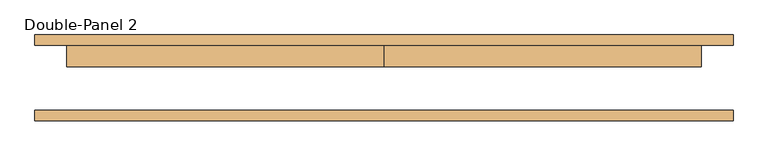
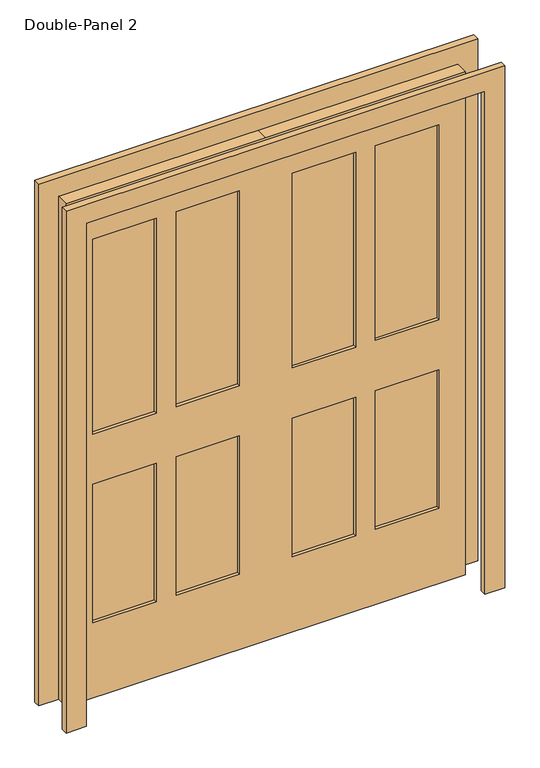
"""IFC4 building model written with IfcOpenShell, lengths in millimetres: door geometry, Double-Panel 2."""

from ifc_helpers import new_model, si_unit, frame, origin, place, context, project, spatial, polyline, outline, extrude, source, transform, mapped, element, save


def double_panel_2_ff76332e(model_context):
    return source(origin(), model_context, "Body", "SweptSolid", [
        extrude(outline(polyline([(2108.2, -838.2), (0.0, -838.2), (0.0, -762.0), (2032.0, -762.0), (2032.0, 762.0), (0.0, 762.0), (0.0, 838.2), (2108.2, 838.2), (2108.2, -838.2)])), frame((0.0, 77.7875, 0.0), z_axis=(0.0, 1.0, 0.0), x_axis=(0.0, 0.0, 1.0)), (0.0, 0.0, 1.0), 25.4),
        extrude(outline(polyline([(419.1, 65.0875), (660.4, 65.0875), (660.4, 39.6875), (419.1, 39.6875), (419.1, 65.0875)])), frame((0.0, 0.0, 1066.8), z_axis=(0.0, 0.0, 1.0), x_axis=(1.0, 0.0, 0.0)), (0.0, 0.0, 1.0), 787.4),
        extrude(outline(polyline([(101.6, 65.0875), (342.9, 65.0875), (342.9, 39.6875), (101.6, 39.6875), (101.6, 65.0875)])), frame((0.0, 0.0, 1066.8), z_axis=(0.0, 0.0, 1.0), x_axis=(1.0, 0.0, 0.0)), (0.0, 0.0, 1.0), 787.4),
        extrude(outline(polyline([(419.1, 65.0875), (660.4, 65.0875), (660.4, 39.6875), (419.1, 39.6875), (419.1, 65.0875)])), frame((0.0, 0.0, 304.8), z_axis=(0.0, 0.0, 1.0), x_axis=(1.0, 0.0, 0.0)), (0.0, 0.0, 1.0), 558.8),
        extrude(outline(polyline([(101.6, 65.0875), (342.9, 65.0875), (342.9, 39.6875), (101.6, 39.6875), (101.6, 65.0875)])), frame((0.0, 0.0, 304.8), z_axis=(0.0, 0.0, 1.0), x_axis=(1.0, 0.0, 0.0)), (0.0, 0.0, 1.0), 558.8),
        extrude(outline(polyline([(-342.9, 65.0875), (-101.6, 65.0875), (-101.6, 39.6875), (-342.9, 39.6875), (-342.9, 65.0875)])), frame((0.0, 0.0, 1066.8), z_axis=(0.0, 0.0, 1.0), x_axis=(1.0, 0.0, 0.0)), (0.0, 0.0, 1.0), 787.4),
        extrude(outline(polyline([(-660.4, 65.0875), (-419.1, 65.0875), (-419.1, 39.6875), (-660.4, 39.6875), (-660.4, 65.0875)])), frame((0.0, 0.0, 1066.8), z_axis=(0.0, 0.0, 1.0), x_axis=(1.0, 0.0, 0.0)), (0.0, 0.0, 1.0), 787.4),
        extrude(outline(polyline([(-342.9, 65.0875), (-101.6, 65.0875), (-101.6, 39.6875), (-342.9, 39.6875), (-342.9, 65.0875)])), frame((0.0, 0.0, 304.8), z_axis=(0.0, 0.0, 1.0), x_axis=(1.0, 0.0, 0.0)), (0.0, 0.0, 1.0), 558.8),
        extrude(outline(polyline([(-660.4, 65.0875), (-419.1, 65.0875), (-419.1, 39.6875), (-660.4, 39.6875), (-660.4, 65.0875)])), frame((0.0, 0.0, 304.8), z_axis=(0.0, 0.0, 1.0), x_axis=(1.0, 0.0, 0.0)), (0.0, 0.0, 1.0), 558.8),
        extrude(outline(polyline([(2032.0, 0.0), (2032.0, -762.0), (0.0, -762.0), (0.0, 0.0), (0.0, 762.0), (2032.0, 762.0), (2032.0, 0.0)]), holes=[polyline([(1854.2, 419.1), (1854.2, 660.4), (1066.8, 660.4), (1066.8, 419.1), (1854.2, 419.1)]), polyline([(1854.2, 101.6), (1854.2, 342.9), (1066.8, 342.9), (1066.8, 101.6), (1854.2, 101.6)]), polyline([(863.6, 419.1), (863.6, 660.4), (304.8, 660.4), (304.8, 419.1), (863.6, 419.1)]), polyline([(863.6, 101.6), (863.6, 342.9), (304.8, 342.9), (304.8, 101.6), (863.6, 101.6)]), polyline([(1066.8, -342.9), (1854.2, -342.9), (1854.2, -101.6), (1066.8, -101.6), (1066.8, -342.9)]), polyline([(1854.2, -660.4), (1854.2, -419.1), (1066.8, -419.1), (1066.8, -660.4), (1854.2, -660.4)]), polyline([(863.6, -342.9), (863.6, -101.6), (304.8, -101.6), (304.8, -342.9), (863.6, -342.9)]), polyline([(863.6, -660.4), (863.6, -419.1), (304.8, -419.1), (304.8, -660.4), (863.6, -660.4)])]), frame((0.0, 26.9875, 0.0), z_axis=(0.0, 1.0, 0.0), x_axis=(0.0, 0.0, 1.0)), (0.0, 0.0, 1.0), 50.8),
        extrude(outline(polyline([(2032.0, -762.0), (2032.0, 762.0), (0.0, 762.0), (0.0, 838.2), (2108.2, 838.2), (2108.2, -838.2), (0.0, -838.2), (0.0, -762.0), (2032.0, -762.0)])), frame((0.0, -103.1875, 0.0), z_axis=(0.0, 1.0, 0.0), x_axis=(0.0, 0.0, 1.0)), (0.0, 0.0, 1.0), 25.4),
    ])


if __name__ == "__main__":
    model = new_model("IFC4")
    model_context = context("Model", 3, world=origin())
    ifc_project = project(units=[si_unit("LENGTHUNIT", "METRE", prefix="MILLI")], contexts=[model_context])
    site = spatial("IfcSite", under=ifc_project)
    building = spatial("IfcBuilding", under=site)
    placement = place(None, origin())
    double_panel_2_shape = double_panel_2_ff76332e(model_context)
    element("IfcDoor", 1, ObjectType="Double-Panel 2 : 60\" x 80\"  White", at=placement, inside=building, context=model_context, shape_type="MappedRepresentation", body=[
        mapped(double_panel_2_shape, transform((0.0, 0.0, 0.0), x_axis=(1.0, 0.0, 0.0), y_axis=(0.0, 1.0, 0.0), z_axis=(0.0, 0.0, 1.0))),
    ])
    save(model, "model.ifc")

# Revit data of these elements
# Type "Double-Panel 2 : 60\" x 80\"  White"
#   Type Mark = "85"
#   COBie.Type.CreatedBy = "doug.wood@us.ibm.com"
#   COBie.Type.CreatedOn = "2016-04-14T02:07:24"
#   COBie.Type.Name = "Doors_Double-Panel 2_60\" x 80\"  White_85"
#   COBie.Type.Category = "23-30 10 00 : Doors"
#   COBie.Type.Description = "Double-Panel 2_60\" x 80\"  White"
#   COBie.Type.Manufacturer = ""
#   COBie.Type.ModelNumber = ""
#   Construction Type Id = "MDOOR"
#   Assembly Code = "C1020"
#   Analytic Construction = "Metal"
#   COBie.Type.ReplacementCost = 0
#   Thickness = 0' - 2"
#   Heat Transfer Coefficient (U) = 3.7021 W/(m²·K)
#   Height = 6' - 8"
#   Trim Projection Ext = 0' - 1"
#   Trim Projection Int = 0' - 1"
#   Trim Width = 0' - 3"
#   Width = 5' - 0"
#   COBie.Type = no
#   Door Material = Door - Panel
#   Frame Material = Trim - White
#   Visual Light Transmittance = 0
#   Solar Heat Gain Coefficient = 0
#   Function = (empty or 0)
#   Wall Closure = (empty or 0)
# Element 1 (IfcDoor, "Double-Panel 2 : 60\" x 80\"  White")
#   Materials on its faces: "Door - Panel", "Trim - White"
# Materials
#   "Door - Panel": class "Wood", colour RGB 255 255 255, transparency 0, Cost = 0
#   "Trim - White": class "Wood", colour RGB 255 255 255, transparency 0, Cost = 0
